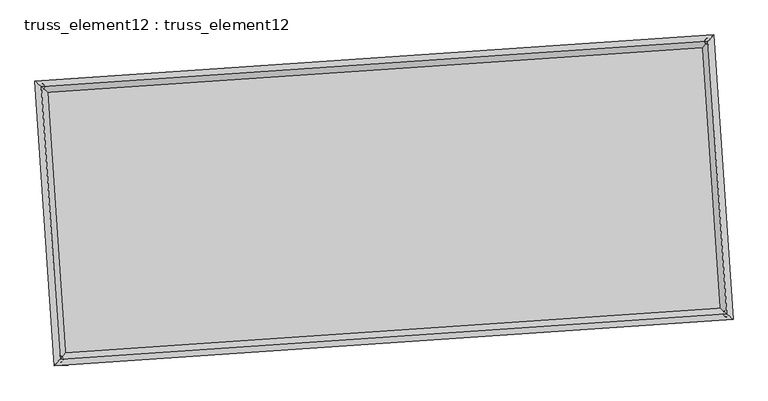
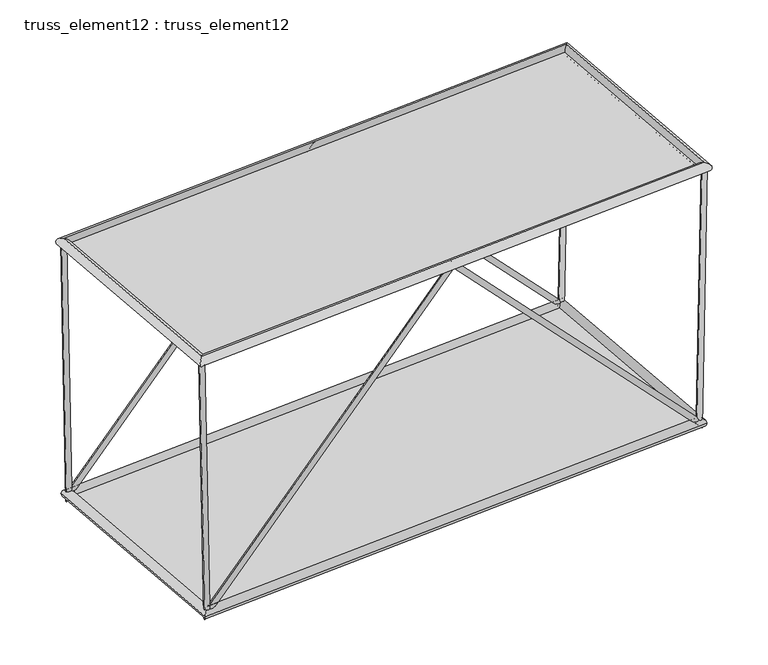
"""IFC4 building model written with IfcOpenShell, lengths in millimetres: plate geometry, truss_element12 : truss_element12."""

from ifc_helpers import new_model, si_unit, frame, origin, origin_with_axes, place, context, project, spatial, polyline, circle_curve, ellipse_curve, outline, extrude, source, transform, mapped, element, save
from ifc_brep_helpers import plane_surface, cylinder_surface, advanced_brep


def truss_element12_truss_element12_8683e9ea(model_context):
    return source(origin(), model_context, "Body", "SolidModel", [
        advanced_brep(
        [(-3763.175469, 2269.5257658, 5000.013006), (-3862.2595379, 2256.1658634, 4998.0482414), (-3667.3230761, 2276.0615761, 121.6864805), (-3761.6638067, 2263.025104, -121.6864805), (1064.4016773, 2598.6999001, 5071.1337295), (1064.8396904, 2592.1260302, 4926.9005993), (5794.7944495, 2921.2474013, 121.6771578), (5889.9665275, 2921.1330872, -121.6771578), (5891.9689049, 2927.8733581, 4999.9996325), (5991.9488375, 2928.0868732, 4998.0077777)],
        [
            (0, 1, circle_curve(frame((-3812.7175034, 2262.8458146, 4999.0306237), z_axis=(-0.019644812406201254, -0.0013395050810558159, 0.9998061247420238), x_axis=(-0.13359944057296166, 0.9910345637327826, -0.0012972916267560764)), 50.0)),
            (1, 0, circle_curve(frame((-3812.7175034, 2262.8458146, 4999.0306237), z_axis=(-0.019644812406201254, -0.0013395050810558159, 0.9998061247420238), x_axis=(-0.13359944057296166, 0.9910345637327826, -0.0012972916267560764)), 50.0)),
            (0, 2),
            (2, 3, ellipse_curve(frame((-3714.4934414, 2269.54334, 0.0), z_axis=(-0.929375267082313, -0.06337056657620804, 0.3636561345935057), x_axis=(0.36281368736471115, 0.0247388861574563, 0.9315332606904114)), 130.9147553, 50.0)),
            (3, 1),
            (3, 2, ellipse_curve(frame((-3714.4934414, 2269.54334, 0.0), z_axis=(-0.929375267082313, -0.06337056657620804, 0.3636561345935057), x_axis=(0.36281368736471115, 0.0247388861574563, 0.9315332606904114)), 130.9147553, 50.0)),
            (2, 4),
            (4, 5, ellipse_curve(frame((1064.6206839, 2595.4129651, 4999.0171644), z_axis=(-0.997683393575001, -0.06802823805824594, 7.079096398493221e-05), x_axis=(-7.062696935952491e-05, -4.815784562580771e-06, -0.9999999974943198)), 72.2735967, 50.0)),
            (5, 3),
            (5, 4, ellipse_curve(frame((1064.6206839, 2595.4129651, 4999.0171644), z_axis=(-0.997683393575001, -0.06802823805824594, 7.079096398493221e-05), x_axis=(-7.062696935952491e-05, -4.815784562580771e-06, -0.9999999974943198)), 72.2735967, 50.0)),
            (4, 6),
            (6, 7, ellipse_curve(frame((5842.3804885, 2921.1902443, 0.0), z_axis=(-0.9294501915680619, -0.06337567539207618, -0.36346370542695344), x_axis=(-0.3626217039803215, -0.024725795540271836, 0.9316083591495455)), 130.8941732, 50.0)),
            (7, 5),
            (7, 6, ellipse_curve(frame((5842.3804885, 2921.1902443, 0.0), z_axis=(-0.9294501915680619, -0.06337567539207618, -0.36346370542695344), x_axis=(-0.3626217039803215, -0.024725795540271836, 0.9316083591495455)), 130.8941732, 50.0)),
            (8, 9, circle_curve(frame((5941.9588712, 2927.9801156, 4999.0037051), z_axis=(0.01991567653237518, 0.0013579742761685913, 0.99980074101499), x_axis=(-0.0021617749268675606, 0.9999967985118469, -0.0013151787796394784)), 50.0)),
            (9, 8, circle_curve(frame((5941.9588712, 2927.9801156, 4999.0037051), z_axis=(0.01991567653237518, 0.0013579742761685913, 0.99980074101499), x_axis=(-0.0021617749268675606, 0.9999967985118469, -0.0013151787796394784)), 50.0)),
            (6, 8),
            (9, 7),
        ],
        [
            plane_surface(frame((-3812.7175034, 2312.8457698, 4999.0976119), z_axis=(-0.019644812406201615, -0.0013395050810550307, 0.9998061247420239), x_axis=(0.9998070220525186, -2.6319405098895743e-05, 0.0196447947753029))),
            cylinder_surface(frame((-3812.7175034, 2262.8458146, 4999.0306237), z_axis=(-0.019644812406201254, -0.0013395050810558159, 0.9998061247420238), x_axis=(-0.13359944057296166, 0.9910345637327826, -0.0012972916267560764)), 50.0),
            cylinder_surface(frame((-3714.4934414, 2269.54334, 0.0), z_axis=(-0.6902639103770004, -0.047066472109834154, -0.7220252635705949), x_axis=(-0.02042044414542879, 0.9987518092655329, -0.04558320907668055)), 50.0),
            cylinder_surface(frame((1064.6206839, 2595.4129651, 4999.0171644), z_axis=(-0.6901619145465986, -0.047059517401881225, 0.722123212153768), x_axis=(-0.11534685580470919, 0.9922791381035594, -0.04557647354090616)), 50.0),
            plane_surface(frame((5941.9588712, 2877.9801618, 4999.0716173), z_axis=(0.019915676532374617, 0.0013579742761693733, 0.99980074101499), x_axis=(0.9998016632453948, -2.705034150096704e-05, -0.019915658161888644))),
            cylinder_surface(frame((5842.3804885, 2921.1902443, 0.0), z_axis=(-0.019915676532375182, -0.0013579742761685915, -0.9998007410149902), x_axis=(-0.0021617749268675606, 0.9999967985118469, -0.0013151787796394784)), 50.0),
        ],
        [
            (0, [[1, 2]]),
            (1, [[-1, 3, 4, 5]]),
            (1, [[-2, -5, 6, -3]]),
            (2, [[-4, 7, 8, 9]]),
            (2, [[-6, -9, 10, -7]]),
            (3, [[-8, 11, 12, 13]]),
            (3, [[-10, -13, 14, -11]]),
            (4, [[15, 16]]),
            (5, [[-12, 17, -16, 18]]),
            (5, [[-14, -18, -15, -17]]),
        ],
    ),
        advanced_brep(
        [(-3491.0625161, -1721.2078185, 5000.013006), (-3590.146585, -1734.5677209, 4998.0482414), (-3395.2101232, -1714.6720082, 121.6864805), (-3489.5508538, -1727.7084803, -121.6864805), (1336.5146302, -1392.0336842, 5071.1337295), (1336.9526433, -1398.6075541, 4926.9005993), (6066.9074025, -1069.486183, 121.6771578), (6162.0794804, -1069.6004971, -121.6771578), (6164.0818578, -1062.8602262, 4999.9996325), (6264.0617904, -1062.6467111, 4998.0077777)],
        [
            (0, 1, circle_curve(frame((-3540.6045505, -1727.8877697, 4999.0306237), z_axis=(-0.0196448124062014, -0.001339505081055837, 0.9998061247420237), x_axis=(-0.1335994405729607, 0.9910345637327829, -0.0012972916267560556)), 50.0)),
            (1, 0, circle_curve(frame((-3540.6045505, -1727.8877697, 4999.0306237), z_axis=(-0.0196448124062014, -0.001339505081055837, 0.9998061247420237), x_axis=(-0.1335994405729607, 0.9910345637327829, -0.0012972916267560556)), 50.0)),
            (0, 2),
            (2, 3, ellipse_curve(frame((-3442.3804885, -1721.1902443, 0.0), z_axis=(-0.929375267082313, -0.06337056657620761, 0.3636561345935053), x_axis=(0.36281368736471076, 0.024738886157456078, 0.9315332606904115)), 130.9147553, 50.0)),
            (3, 1),
            (3, 2, ellipse_curve(frame((-3442.3804885, -1721.1902443, 0.0), z_axis=(-0.929375267082313, -0.06337056657620761, 0.3636561345935053), x_axis=(0.36281368736471076, 0.024738886157456078, 0.9315332606904115)), 130.9147553, 50.0)),
            (2, 4),
            (4, 5, ellipse_curve(frame((1336.7336368, -1395.3206192, 4999.0171644), z_axis=(-0.9976833935750008, -0.06802823805824576, 7.079096398437052e-05), x_axis=(-7.062696935952493e-05, -4.815784562254043e-06, -0.9999999974943198)), 72.2735967, 50.0)),
            (5, 3),
            (5, 4, ellipse_curve(frame((1336.7336368, -1395.3206192, 4999.0171644), z_axis=(-0.9976833935750008, -0.06802823805824576, 7.079096398437052e-05), x_axis=(-7.062696935952493e-05, -4.815784562254043e-06, -0.9999999974943198)), 72.2735967, 50.0)),
            (4, 6),
            (6, 7, ellipse_curve(frame((6114.4934414, -1069.54334, 0.0), z_axis=(-0.9294501915680616, -0.06337567539207624, -0.3634637054269544), x_axis=(-0.36262170398032223, -0.024725795540271968, 0.9316083591495453)), 130.8941732, 50.0)),
            (7, 5),
            (7, 6, ellipse_curve(frame((6114.4934414, -1069.54334, 0.0), z_axis=(-0.9294501915680616, -0.06337567539207624, -0.3634637054269544), x_axis=(-0.36262170398032223, -0.024725795540271968, 0.9316083591495453)), 130.8941732, 50.0)),
            (8, 9, circle_curve(frame((6214.0718241, -1062.7534687, 4999.0037051), z_axis=(0.0199156765323745, 0.0013579742761685016, 0.9998007410149902), x_axis=(-0.0021617749268679704, 0.9999967985118469, -0.0013151787796393817)), 50.0)),
            (9, 8, circle_curve(frame((6214.0718241, -1062.7534687, 4999.0037051), z_axis=(0.0199156765323745, 0.0013579742761685016, 0.9998007410149902), x_axis=(-0.0021617749268679704, 0.9999967985118469, -0.0013151787796393817)), 50.0)),
            (6, 8),
            (9, 7),
        ],
        [
            plane_surface(frame((-3540.6045505, -1677.8878145, 4999.0976119), z_axis=(-0.019644812406201615, -0.0013395050810550307, 0.9998061247420239), x_axis=(0.9998070220525186, -2.6319405098895743e-05, 0.0196447947753029))),
            cylinder_surface(frame((-3540.6045505, -1727.8877697, 4999.0306237), z_axis=(-0.019644812406201403, -0.0013395050810558371, 0.9998061247420239), x_axis=(-0.1335994405729607, 0.9910345637327829, -0.0012972916267560556)), 50.0),
            cylinder_surface(frame((-3442.3804885, -1721.1902443, 0.0), z_axis=(-0.6902639103769999, -0.04706647210983376, -0.7220252635705952), x_axis=(-0.02042044414542852, 0.9987518092655328, -0.04558320907668025)), 50.0),
            cylinder_surface(frame((1336.7336368, -1395.3206192, 4999.0171644), z_axis=(-0.6901619145465989, -0.04705951740188135, 0.7221232121537675), x_axis=(-0.11534685580470896, 0.9922791381035595, -0.045576473540905854)), 50.0),
            plane_surface(frame((6214.0718241, -1112.7534225, 4999.0716173), z_axis=(0.019915676532374617, 0.001357974276169373, 0.99980074101499), x_axis=(0.9998016632453948, -2.7050341500522952e-05, -0.019915658161888644))),
            cylinder_surface(frame((6114.4934414, -1069.54334, 0.0), z_axis=(-0.0199156765323745, -0.0013579742761685016, -0.9998007410149902), x_axis=(-0.0021617749268679704, 0.9999967985118469, -0.0013151787796393817)), 50.0),
        ],
        [
            (0, [[1, 2]]),
            (1, [[-1, 3, 4, 5]]),
            (1, [[-2, -5, 6, -3]]),
            (2, [[-4, 7, 8, 9]]),
            (2, [[-6, -9, 10, -7]]),
            (3, [[-8, 11, 12, 13]]),
            (3, [[-10, -13, 14, -11]]),
            (4, [[15, 16]]),
            (5, [[-12, 17, -16, 18]]),
            (5, [[-14, -18, -15, -17]]),
        ],
    ),
        advanced_brep(
        [(-3540.6115622, -1727.895541, 4909.030624), (-3540.5975388, -1727.8799983, 5089.0306234), (-3812.7095018, 2262.839067, 5089.0306234), (-3812.7255051, 2262.8525623, 4909.030624), (5941.9523539, 2927.972378, 5089.0037048), (5941.9653884, 2927.9878533, 4909.0037053), (6214.0643168, -1062.7466873, 5089.0037048), (6214.0793313, -1062.76025, 4909.0037053)],
        [
            (0, 1, ellipse_curve(frame((-3540.6045505, -1727.8877697, 4999.0306237), z_axis=(-0.7535719234027833, 0.6573654662782641, 1.9467846704927456e-06), x_axis=(-0.657365466275408, -0.7535719234052748, 1.9467846704929505e-06)), 127.2792206, 90.0)),
            (1, 2),
            (2, 3, ellipse_curve(frame((-3812.7175034, 2262.8458146, 4999.0306237), z_axis=(-0.6573654662754078, -0.7535719234052749, 1.9467846704931415e-06), x_axis=(0.7535719234027833, -0.6573654662782641, -1.946784670492937e-06)), 127.2792206, 90.0)),
            (3, 0),
            (1, 0, ellipse_curve(frame((-3540.6045505, -1727.8877697, 4999.0306237), z_axis=(-0.7535719234027833, 0.6573654662782641, 1.9467846704927456e-06), x_axis=(-0.657365466275408, -0.7535719234052748, 1.9467846704929505e-06)), 127.2792206, 90.0)),
            (3, 2, ellipse_curve(frame((-3812.7175034, 2262.8458146, 4999.0306237), z_axis=(-0.6573654662754078, -0.7535719234052749, 1.9467846704931415e-06), x_axis=(0.7535719234027833, -0.6573654662782641, -1.946784670492937e-06)), 127.2792206, 90.0)),
            (2, 4),
            (4, 5, ellipse_curve(frame((5941.9588712, 2927.9801156, 4999.0037051), z_axis=(-0.7535719234027835, 0.6573654662782641, 1.94678467049313e-06), x_axis=(-0.6573654662754079, -0.7535719234052748, 1.9467846704929493e-06)), 127.2792206, 90.0)),
            (5, 3),
            (5, 4, ellipse_curve(frame((5941.9588712, 2927.9801156, 4999.0037051), z_axis=(-0.7535719234027835, 0.6573654662782641, 1.94678467049313e-06), x_axis=(-0.6573654662754079, -0.7535719234052748, 1.9467846704929493e-06)), 127.2792206, 90.0)),
            (4, 6),
            (6, 7, ellipse_curve(frame((6214.0718241, -1062.7534687, 4999.0037051), z_axis=(0.6573654662754082, 0.7535719234052746, -1.9467846704927583e-06), x_axis=(-0.7535719234027829, 0.6573654662782644, 1.946784670492937e-06)), 127.2792206, 90.0)),
            (7, 5),
            (7, 6, ellipse_curve(frame((6214.0718241, -1062.7534687, 4999.0037051), z_axis=(0.6573654662754082, 0.7535719234052746, -1.9467846704927583e-06), x_axis=(-0.7535719234027829, 0.6573654662782644, 1.946784670492937e-06)), 127.2792206, 90.0)),
            (6, 1),
            (0, 7),
        ],
        [
            cylinder_surface(frame((-3540.6045505, -1727.8877697, 4999.0306237), z_axis=(0.06802823822870033, -0.9976833960748768, 0.0), x_axis=(-0.9976833925883778, -0.06802823799096921, 8.360136848613292e-05)), 90.0),
            cylinder_surface(frame((-3812.7175034, 2262.8458146, 4999.0306237), z_axis=(-0.9976833960710954, -0.06802823822844235, 2.7531692840312938e-06), x_axis=(-0.0680282377842961, 0.9976833928293745, 8.084819921109972e-05)), 90.0),
            cylinder_surface(frame((5941.9588712, 2927.9801156, 4999.0037051), z_axis=(-0.06802823822869988, 0.9976833960748767, 0.0), x_axis=(0.9976833930325241, 0.06802823802125342, 7.809502993606649e-05)), 90.0),
            cylinder_surface(frame((6214.0718241, -1062.7534687, 4999.0037051), z_axis=(0.9976833960710956, 0.06802823822844176, -2.753169284031023e-06), x_axis=(0.06802823822844174, -0.9976833927990899, 8.084819921109968e-05)), 90.0),
        ],
        [
            (0, [[1, 2, 3, 4]]),
            (0, [[5, -4, 6, -2]]),
            (1, [[-3, 7, 8, 9]]),
            (1, [[-6, -9, 10, -7]]),
            (2, [[-8, 11, 12, 13]]),
            (2, [[-10, -13, 14, -11]]),
            (3, [[-12, 15, -1, 16]]),
            (3, [[-14, -16, -5, -15]]),
        ],
    ),
        advanced_brep(
        [(-3358.7115243, -1625.2761972, 0.0), (-3526.0494527, -1817.1042913, 0.0), (-3810.4074885, 2353.2123043, 0.0), (-3618.5793943, 2185.8743758, 0.0), (5926.0494527, 3017.1042913, 0.0), (5758.7115243, 2825.2761972, 0.0), (6210.4074885, -1153.2123043, 0.0), (6018.5793943, -985.8743758, 0.0)],
        [
            (0, 1, ellipse_curve(frame((-3442.3804885, -1721.1902443, 0.0), z_axis=(-0.7535719234054589, 0.6573654662780799, 0.0), x_axis=(-0.65736546627808, -0.7535719234054586, 0.0)), 127.2792206, 90.0)),
            (1, 2),
            (2, 3, ellipse_curve(frame((-3714.4934414, 2269.54334, 0.0), z_axis=(-0.6573654662780796, -0.7535719234054589, 0.0), x_axis=(0.7535719234054588, -0.6573654662780798, 0.0)), 127.2792206, 90.0)),
            (3, 0),
            (1, 0, ellipse_curve(frame((-3442.3804885, -1721.1902443, 0.0), z_axis=(-0.7535719234054589, 0.6573654662780799, 0.0), x_axis=(-0.65736546627808, -0.7535719234054586, 0.0)), 127.2792206, 90.0)),
            (3, 2, ellipse_curve(frame((-3714.4934414, 2269.54334, 0.0), z_axis=(-0.6573654662780796, -0.7535719234054589, 0.0), x_axis=(0.7535719234054588, -0.6573654662780798, 0.0)), 127.2792206, 90.0)),
            (2, 4),
            (4, 5, ellipse_curve(frame((5842.3804885, 2921.1902443, 0.0), z_axis=(-0.7535719234054588, 0.6573654662780799, 0.0), x_axis=(-0.6573654662780799, -0.7535719234054586, 0.0)), 127.2792206, 90.0)),
            (5, 3),
            (5, 4, ellipse_curve(frame((5842.3804885, 2921.1902443, 0.0), z_axis=(-0.7535719234054588, 0.6573654662780799, 0.0), x_axis=(-0.6573654662780799, -0.7535719234054586, 0.0)), 127.2792206, 90.0)),
            (4, 6),
            (6, 7, ellipse_curve(frame((6114.4934414, -1069.54334, 0.0), z_axis=(0.65736546627808, 0.7535719234054586, 0.0), x_axis=(-0.7535719234054585, 0.6573654662780801, 0.0)), 127.2792206, 90.0)),
            (7, 5),
            (7, 6, ellipse_curve(frame((6114.4934414, -1069.54334, 0.0), z_axis=(0.65736546627808, 0.7535719234054586, 0.0), x_axis=(-0.7535719234054585, 0.6573654662780801, 0.0)), 127.2792206, 90.0)),
            (6, 1),
            (0, 7),
        ],
        [
            cylinder_surface(frame((-3442.3804885, -1721.1902443, 0.0), z_axis=(0.06802823822870284, -0.9976833960748764, 0.0), x_axis=(-0.9976833960748764, -0.06802823822870284, 0.0)), 90.0),
            cylinder_surface(frame((-3714.4934414, 2269.54334, 0.0), z_axis=(-0.9976833960748764, -0.06802823822870264, 0.0), x_axis=(-0.06802823822870264, 0.9976833960748764, 0.0)), 90.0),
            cylinder_surface(frame((5842.3804885, 2921.1902443, 0.0), z_axis=(-0.06802823822870245, 0.9976833960748767, 0.0), x_axis=(0.9976833960748767, 0.06802823822870245, 0.0)), 90.0),
            cylinder_surface(frame((6114.4934414, -1069.54334, 0.0), z_axis=(0.9976833960748767, 0.0680282382287021, 0.0), x_axis=(0.0680282382287021, -0.9976833960748767, 0.0)), 90.0),
        ],
        [
            (0, [[1, 2, 3, 4]]),
            (0, [[5, -4, 6, -2]]),
            (1, [[-3, 7, 8, 9]]),
            (1, [[-6, -9, 10, -7]]),
            (2, [[-8, 11, 12, 13]]),
            (2, [[-10, -13, 14, -11]]),
            (3, [[-12, 15, -1, 16]]),
            (3, [[-14, -16, -5, -15]]),
        ],
    ),
        extrude(outline(polyline([(-3442.3804885, -1721.1902443), (-3714.4934414, 2269.54334), (5842.3804885, 2921.1902443), (6114.4934414, -1069.54334), (-3442.3804885, -1721.1902443)])), origin_with_axes(), (0.0, 0.0, 1.0), 20.0),
        extrude(outline(polyline([(-2000.0000001, 4888.6632838), (1999.9999999, 4888.6632838), (2000.0, -4888.6632839), (-2000.0, -4888.6632839), (-2000.0000001, 4888.6632838)])), frame((1200.6771603, 600.046173, 4999.0171644), z_axis=(2.7467912812612416e-06, 1.8729325593801917e-07, 0.99999999999621), x_axis=(-0.06802823822870298, 0.9976833960748764, 0.0)), (0.0, 0.0, 1.0), 20.0),
    ])


if __name__ == "__main__":
    model = new_model("IFC4")
    model_context = context("Model", 3, world=origin())
    ifc_project = project(units=[si_unit("LENGTHUNIT", "METRE", prefix="MILLI")], contexts=[model_context])
    site = spatial("IfcSite", under=ifc_project)
    building = spatial("IfcBuilding", under=site)
    placement = place(None, origin())
    truss_element12_truss_element12_shape = truss_element12_truss_element12_8683e9ea(model_context)
    element("IfcPlate", 1, ObjectType="truss_element12 : truss_element12", at=placement, inside=building, context=model_context, shape_type="MappedRepresentation", body=[
        mapped(truss_element12_truss_element12_shape, transform((0.0, 0.0, 0.0), x_axis=(1.0, 0.0, 0.0), y_axis=(0.0, 1.0, 0.0), z_axis=(0.0, 0.0, 1.0))),
    ])
    save(model, "model.ifc")

# Revit data of these elements
# Type "truss_element12 : truss_element12"
#   steellbar1 = 90 mm
#   steelbar2 = 50 mm
#   offset1 = 5000 mm
#   M = Default Roof
# Element 1 (IfcPlate, "truss_element12 : truss_element12")
#   Materials on its faces: "Default Roof"
# Materials
#   "Default Roof": class "Miscellaneous", colour RGB 0 127 0, transparency 0, Comments = "Rendering appearance not upgraded Rendering appearance not upgraded ", Cost = 0
